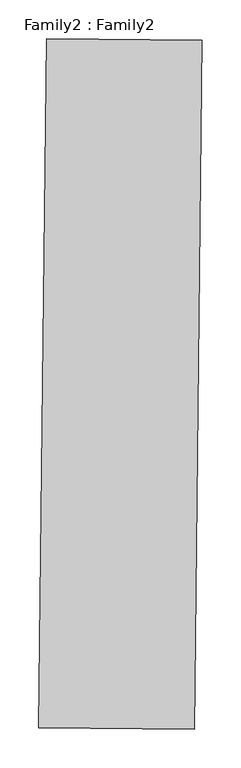
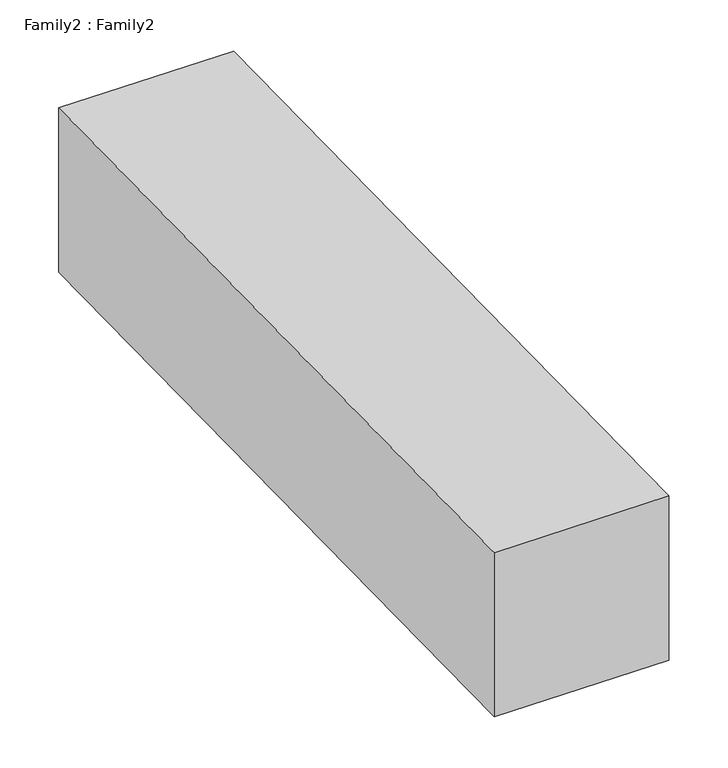
"""IFC4 building model written with IfcOpenShell, lengths in millimetres: proxy geometry, Family2 : Family2."""

from ifc_helpers import new_model, si_unit, origin, place, context, project, spatial, faceted_brep, source, transform, mapped, element, save


def family2_family2_caec7af3(model_context):
    return source(origin(), model_context, "Body", "Brep", [
        faceted_brep([(-3948.3898749, -6516.3415583, 1.0945136), (-3948.3898749, -6516.3415583, 201.0945136), (-3938.4529196, -5631.2585643, 202.060409), (-3938.4529196, -5631.2585643, 2.060409), (-3748.3986849, -6518.2187709, 201.0945136), (-3738.4617297, -5633.135777, 202.060409), (-3748.3986849, -6518.2187709, 1.0945136), (-3738.4617297, -5633.135777, 2.060409)], [[[0, 1, 2, 3]], [[1, 4, 5, 2]], [[4, 6, 7, 5]], [[6, 0, 3, 7]], [[3, 2, 5, 7]], [[0, 6, 4, 1]]]),
    ])


if __name__ == "__main__":
    model = new_model("IFC4")
    model_context = context("Model", 3, world=origin())
    ifc_project = project(units=[si_unit("LENGTHUNIT", "METRE", prefix="MILLI")], contexts=[model_context])
    site = spatial("IfcSite", under=ifc_project)
    building = spatial("IfcBuilding", under=site)
    placement = place(None, origin())
    family2_family2_shape = family2_family2_caec7af3(model_context)
    element("IfcBuildingElementProxy", 1, Name="Family2 : Family2", ObjectType="Family2 : Family2", at=placement, inside=building, context=model_context, shape_type="MappedRepresentation", body=[
        mapped(family2_family2_shape, transform((0.0, 0.0, 0.0), x_axis=(1.0, 0.0, 0.0), y_axis=(0.0, 1.0, 0.0), z_axis=(0.0, 0.0, 1.0))),
    ])
    save(model, "model.ifc")

# Revit data of these elements
# Type "Family2 : Family2"
#   Default Elevation = 0
